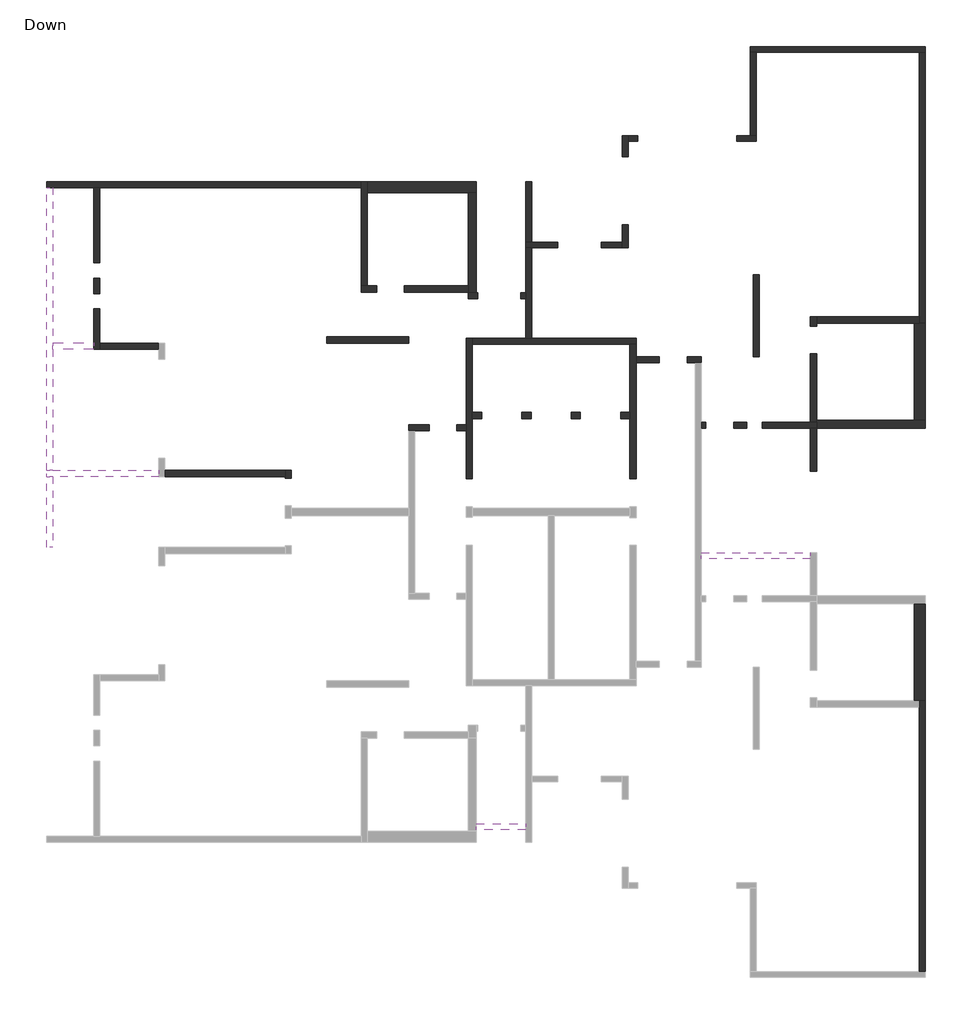
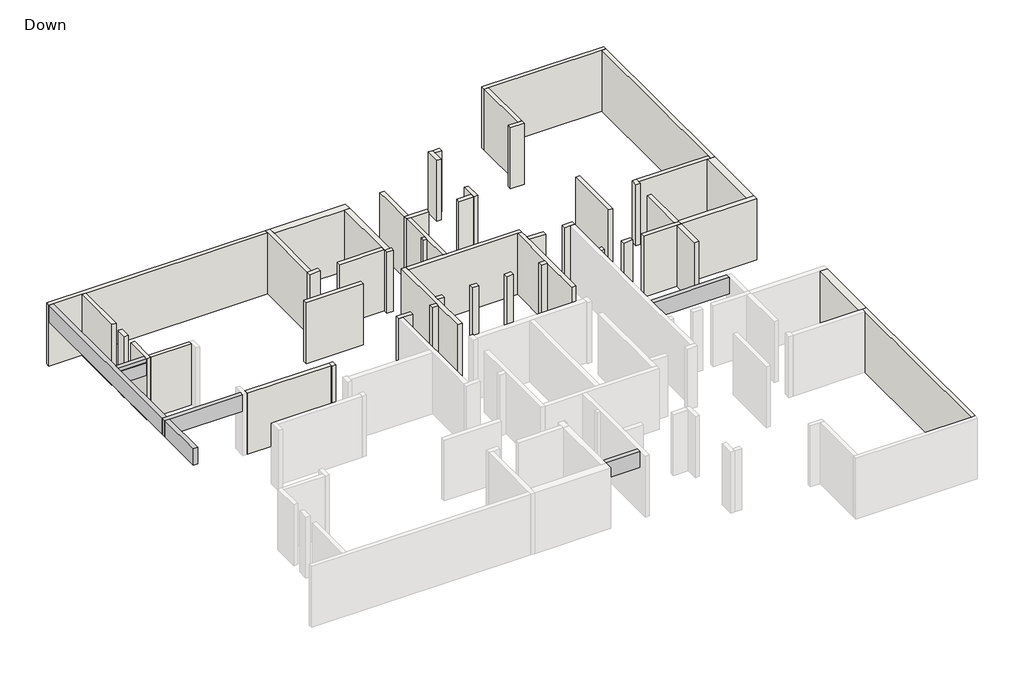
# One storey, part 2 of 2: 49 walls, 6 beams.
# Revit data of these elements (continued)
# Element 5 (IfcBeam, "Concrete Rectengular Beam : 20/80") (continued)
#   Comments = ""
#   Mark = "B8"
#   SOFiSTiK_AMG_Comments = ""
#   SOFiSTiK_AMG_Scheduled = yes
#   SOFiSTiK_AMG_Adjusted = yes
#   Structural Material = Concrete
#   Phase Created = New Construction
#   Materials on its faces: "Concrete"
# Element 6 (IfcBeam, "Concrete Rectengular Beam : 20/80")
#   Comments = ""
#   Mark = "B9"
#   SOFiSTiK_AMG_Comments = ""
#   SOFiSTiK_AMG_Scheduled = yes
#   SOFiSTiK_AMG_Adjusted = yes
#   Structural Material = Concrete
#   Phase Created = New Construction
#   Materials on its faces: "Concrete"
# Element 7 (IfcWall, "19")
#   Comments = ""
#   Mark = "W1"
#   SOFiSTiK_EdgeZones = "W1"
#   SOFiSTiK_AMG_Comments = ""
#   Top Offset = 0 cm
#   Base Offset = 0 cm
#   wall height = 300 cm
#   SOFiSTiK_AMG_Scheduled = yes
#   SOFiSTiK_AMG_Adjusted = yes
#   Phase Created = New Construction
#   Base Constraint = Down
#   Top Constraint = Typical Floor
#   Materials on its faces: "Concrete"
# Element 8 (IfcWall, "19")
#   Comments = ""
#   Mark = "W2"
#   SOFiSTiK_EdgeZones = "W2"
#   SOFiSTiK_AMG_Comments = ""
#   Top Offset = 0 cm
#   Base Offset = 0 cm
#   wall height = 300 cm
#   SOFiSTiK_AMG_Scheduled = yes
#   SOFiSTiK_AMG_Adjusted = yes
#   Phase Created = New Construction
#   Base Constraint = Down
#   Top Constraint = Typical Floor
#   Materials on its faces: "Concrete"
# Element 9 (IfcWall, "19")
#   Comments = ""
#   Mark = "W3"
#   SOFiSTiK_EdgeZones = "W3"
#   SOFiSTiK_AMG_Comments = ""
#   Top Offset = 0 cm
#   Base Offset = 0 cm
#   wall height = 300 cm
#   SOFiSTiK_AMG_Scheduled = yes
#   SOFiSTiK_AMG_Adjusted = yes
#   Phase Created = New Construction
#   Base Constraint = Down
#   Top Constraint = Typical Floor
#   Materials on its faces: "Concrete"
# Element 10 (IfcWall, "19")
#   Comments = ""
#   Mark = "W4"
#   SOFiSTiK_EdgeZones = "W4"
#   SOFiSTiK_AMG_Comments = ""
#   Top Offset = 0 cm
#   Base Offset = 0 cm
#   wall height = 300 cm
#   SOFiSTiK_AMG_Scheduled = yes
#   SOFiSTiK_AMG_Adjusted = yes
#   Phase Created = New Construction
#   Base Constraint = Down
#   Top Constraint = Typical Floor
#   Materials on its faces: "Concrete"
# Element 11 (IfcWall, "19")
#   Comments = ""
#   Mark = "W5"
#   SOFiSTiK_EdgeZones = "W5"
#   SOFiSTiK_AMG_Comments = ""
#   Top Offset = 0 cm
#   Base Offset = 0 cm
#   wall height = 300 cm
#   SOFiSTiK_AMG_Scheduled = yes
#   SOFiSTiK_AMG_Adjusted = yes
#   Phase Created = New Construction
#   Base Constraint = Down
#   Top Constraint = Typical Floor
#   Materials on its faces: "Concrete"
# Element 12 (IfcWall, "19")
#   Comments = ""
#   Mark = "W6"
#   SOFiSTiK_EdgeZones = "W6"
#   SOFiSTiK_AMG_Comments = ""
#   Top Offset = 0 cm
#   Base Offset = 0 cm
#   wall height = 300 cm
#   SOFiSTiK_AMG_Scheduled = yes
#   SOFiSTiK_AMG_Adjusted = yes
#   Phase Created = New Construction
#   Base Constraint = Down
#   Top Constraint = Typical Floor
#   Materials on its faces: "Concrete"
# Element 13 (IfcWall, "19")
#   Comments = ""
#   Mark = "W7"
#   SOFiSTiK_EdgeZones = "W7"
#   SOFiSTiK_AMG_Comments = ""
#   Top Offset = 0 cm
#   Base Offset = 0 cm
#   wall height = 300 cm
#   SOFiSTiK_AMG_Scheduled = yes
#   SOFiSTiK_AMG_Adjusted = yes
#   Phase Created = New Construction
#   Base Constraint = Down
#   Top Constraint = Typical Floor
#   Materials on its faces: "Concrete"
# Element 14 (IfcWall, "19")
#   Comments = ""
#   Mark = "W8"
#   SOFiSTiK_EdgeZones = "W8"
#   SOFiSTiK_AMG_Comments = ""
#   Top Offset = 0 cm
#   Base Offset = 0 cm
#   wall height = 300 cm
#   SOFiSTiK_AMG_Scheduled = yes
#   SOFiSTiK_AMG_Adjusted = yes
#   Phase Created = New Construction
#   Base Constraint = Down
#   Top Constraint = Typical Floor
#   Materials on its faces: "Concrete"
# Element 15 (IfcWall, "19")
#   Comments = ""
#   Mark = "W9"
#   SOFiSTiK_EdgeZones = "W9"
#   SOFiSTiK_AMG_Comments = ""
#   Top Offset = 0 cm
#   Base Offset = 0 cm
#   wall height = 300 cm
#   SOFiSTiK_AMG_Scheduled = yes
#   SOFiSTiK_AMG_Adjusted = yes
#   Phase Created = New Construction
#   Base Constraint = Down
#   Top Constraint = Typical Floor
#   Materials on its faces: "Concrete"
# Element 16 (IfcWall, "19")
#   Comments = ""
#   Mark = "W10"
#   SOFiSTiK_EdgeZones = "W10"
#   SOFiSTiK_AMG_Comments = ""
#   Top Offset = 0 cm
#   Base Offset = 0 cm
#   wall height = 300 cm
#   SOFiSTiK_AMG_Scheduled = yes
#   SOFiSTiK_AMG_Adjusted = yes
#   Phase Created = New Construction
#   Base Constraint = Down
#   Top Constraint = Typical Floor
#   Materials on its faces: "Concrete"
# Element 17 (IfcWall, "19")
#   Comments = ""
#   Mark = "W11"
#   SOFiSTiK_EdgeZones = "W11"
#   SOFiSTiK_AMG_Comments = ""
#   Top Offset = 0 cm
#   Base Offset = 0 cm
#   wall height = 300 cm
#   SOFiSTiK_AMG_Scheduled = yes
#   SOFiSTiK_AMG_Adjusted = yes
#   Phase Created = New Construction
#   Base Constraint = Down
#   Top Constraint = Typical Floor
#   Materials on its faces: "Concrete"
# Element 18 (IfcWall, "19")
#   Comments = ""
#   Mark = "W12"
#   SOFiSTiK_EdgeZones = "W12"
#   SOFiSTiK_AMG_Comments = ""
#   Top Offset = 0 cm
#   Base Offset = 0 cm
#   wall height = 300 cm
#   SOFiSTiK_AMG_Scheduled = yes
#   SOFiSTiK_AMG_Adjusted = yes
#   Phase Created = New Construction
#   Base Constraint = Down
#   Top Constraint = Typical Floor
#   Materials on its faces: "Concrete"
# Element 19 (IfcWall, "19")
#   Comments = ""
#   Mark = "W13"
#   SOFiSTiK_EdgeZones = "W13"
#   SOFiSTiK_AMG_Comments = ""
#   Top Offset = 0 cm
#   Base Offset = 0 cm
#   wall height = 300 cm
#   SOFiSTiK_AMG_Scheduled = yes
#   SOFiSTiK_AMG_Adjusted = yes
#   Phase Created = New Construction
#   Base Constraint = Down
#   Top Constraint = Typical Floor
#   Materials on its faces: "Concrete"
# Element 20 (IfcWall, "19")
#   Comments = ""
#   Mark = "W14"
#   SOFiSTiK_EdgeZones = "W14"
#   SOFiSTiK_AMG_Comments = ""
#   Top Offset = 0 cm
#   Base Offset = 0 cm
#   wall height = 300 cm
#   SOFiSTiK_AMG_Scheduled = yes
#   SOFiSTiK_AMG_Adjusted = yes
#   Phase Created = New Construction
#   Base Constraint = Down
#   Top Constraint = Typical Floor
#   Materials on its faces: "Concrete"
# Element 21 (IfcWall, "19")
#   Comments = ""
#   Mark = "W15"
#   SOFiSTiK_EdgeZones = "W15"
#   SOFiSTiK_AMG_Comments = ""
#   Top Offset = 0 cm
#   Base Offset = 0 cm
#   wall height = 300 cm
#   SOFiSTiK_AMG_Scheduled = yes
#   SOFiSTiK_AMG_Adjusted = yes
#   Phase Created = New Construction
#   Base Constraint = Down
#   Top Constraint = Typical Floor
#   Materials on its faces: "Concrete"
# Element 22 (IfcWall, "19")
#   Comments = ""
#   Mark = "W18"
#   SOFiSTiK_EdgeZones = "W18"
#   SOFiSTiK_AMG_Comments = ""
#   Top Offset = 0 cm
#   Base Offset = 0 cm
#   wall height = 300 cm
#   SOFiSTiK_AMG_Scheduled = yes
#   SOFiSTiK_AMG_Adjusted = yes
#   Phase Created = New Construction
#   Base Constraint = Down
#   Top Constraint = Typical Floor
#   Materials on its faces: "Concrete"
# Element 23 (IfcWall, "19")
#   Comments = ""
#   Mark = "W20"
#   SOFiSTiK_EdgeZones = "W20"
#   SOFiSTiK_AMG_Comments = ""
#   Top Offset = 0 cm
#   Base Offset = 0 cm
#   wall height = 300 cm
#   SOFiSTiK_AMG_Scheduled = yes
#   SOFiSTiK_AMG_Adjusted = yes
#   Phase Created = New Construction
#   Base Constraint = Down
#   Top Constraint = Typical Floor
#   Materials on its faces: "Concrete"
# Element 24 (IfcWall, "19")
#   Comments = ""
#   Mark = "W21"
#   SOFiSTiK_EdgeZones = "W21"
#   SOFiSTiK_AMG_Comments = ""
#   Top Offset = 0 cm
#   Base Offset = 0 cm
#   wall height = 300 cm
#   SOFiSTiK_AMG_Scheduled = yes
#   SOFiSTiK_AMG_Adjusted = yes
#   Phase Created = New Construction
#   Base Constraint = Down
#   Top Constraint = Typical Floor
#   Materials on its faces: "Concrete"
# Element 25 (IfcWall, "19")
#   Comments = ""
#   Mark = "W22"
#   SOFiSTiK_EdgeZones = "W22"
#   SOFiSTiK_AMG_Comments = ""
#   Top Offset = 0 cm
#   Base Offset = 0 cm
#   wall height = 300 cm
#   SOFiSTiK_AMG_Scheduled = yes
#   SOFiSTiK_AMG_Adjusted = yes
#   Phase Created = New Construction
#   Base Constraint = Down
#   Top Constraint = Typical Floor
#   Materials on its faces: "Concrete"
# Element 26 (IfcWall, "19")
#   Comments = ""
#   Mark = "W36"
#   SOFiSTiK_EdgeZones = "W36"
#   SOFiSTiK_AMG_Comments = ""
#   Top Offset = 0 cm
#   Base Offset = 0 cm
#   wall height = 300 cm
#   SOFiSTiK_AMG_Scheduled = yes
#   SOFiSTiK_AMG_Adjusted = yes
#   Phase Created = New Construction
#   Base Constraint = Down
#   Top Constraint = Typical Floor
#   Materials on its faces: "Concrete"
# Element 27 (IfcWall, "20")
#   Comments = ""
#   Mark = "W44"
#   SOFiSTiK_EdgeZones = "W44"
#   SOFiSTiK_AMG_Comments = ""
#   Top Offset = 0 cm
#   Base Offset = 0 cm
#   wall height = 300 cm
#   SOFiSTiK_AMG_Scheduled = yes
#   SOFiSTiK_AMG_Adjusted = yes
#   Phase Created = New Construction
#   Base Constraint = Down
#   Top Constraint = Typical Floor
#   Materials on its faces: "Concrete"
# Element 28 (IfcWall, "20")
#   Comments = ""
#   Mark = "W45"
#   SOFiSTiK_EdgeZones = "W45"
#   SOFiSTiK_AMG_Comments = ""
#   Top Offset = 0 cm
#   Base Offset = 0 cm
#   wall height = 300 cm
#   SOFiSTiK_AMG_Scheduled = yes
#   SOFiSTiK_AMG_Adjusted = yes
#   Phase Created = New Construction
#   Base Constraint = Down
#   Top Constraint = Typical Floor
#   Materials on its faces: "Concrete"
# Element 29 (IfcWall, "20")
#   Comments = ""
#   Mark = "W46"
#   SOFiSTiK_EdgeZones = "W46"
#   SOFiSTiK_AMG_Comments = ""
#   Top Offset = 0 cm
#   Base Offset = 0 cm
#   wall height = 300 cm
#   SOFiSTiK_AMG_Scheduled = yes
#   SOFiSTiK_AMG_Adjusted = yes
#   Phase Created = New Construction
#   Base Constraint = Down
#   Top Constraint = Typical Floor
#   Materials on its faces: "Concrete"
# Element 30 (IfcWall, "20")
#   Comments = ""
#   Mark = "W47"
#   SOFiSTiK_EdgeZones = "W47"
#   SOFiSTiK_AMG_Comments = ""
#   Top Offset = 0 cm
#   Base Offset = 0 cm
#   wall height = 300 cm
#   SOFiSTiK_AMG_Scheduled = yes
#   SOFiSTiK_AMG_Adjusted = yes
#   Phase Created = New Construction
#   Base Constraint = Down
#   Top Constraint = Typical Floor
#   Materials on its faces: "Concrete"
# Element 31 (IfcWall, "20")
#   Comments = ""
#   Mark = "W48"
#   SOFiSTiK_EdgeZones = "W48"
#   SOFiSTiK_AMG_Comments = ""
#   Top Offset = 0 cm
#   Base Offset = 0 cm
#   wall height = 300 cm
#   SOFiSTiK_AMG_Scheduled = yes
#   SOFiSTiK_AMG_Adjusted = yes
#   Phase Created = New Construction
#   Base Constraint = Down
#   Top Constraint = Typical Floor
#   Materials on its faces: "Concrete"
# Element 32 (IfcWall, "20")
#   Comments = ""
#   Mark = "W49"
#   SOFiSTiK_EdgeZones = "W49"
#   SOFiSTiK_AMG_Comments = ""
#   Top Offset = 0 cm
#   Base Offset = 0 cm
#   wall height = 300 cm
#   SOFiSTiK_AMG_Scheduled = yes
#   SOFiSTiK_AMG_Adjusted = yes
#   Phase Created = New Construction
#   Base Constraint = Down
#   Top Constraint = Typical Floor
#   Materials on its faces: "Concrete"
# Element 33 (IfcWall, "20")
#   Comments = ""
#   Mark = "W51"
#   SOFiSTiK_EdgeZones = "W51"
#   SOFiSTiK_AMG_Comments = ""
#   Top Offset = 0 cm
#   Base Offset = 0 cm
#   wall height = 300 cm
#   SOFiSTiK_AMG_Scheduled = yes
#   SOFiSTiK_AMG_Adjusted = yes
#   Phase Created = New Construction
#   Base Constraint = Down
#   Top Constraint = Typical Floor
#   Materials on its faces: "Concrete"
# Element 34 (IfcWall, "20")
#   Comments = ""
#   Mark = "W52"
#   SOFiSTiK_EdgeZones = "W52"
#   SOFiSTiK_AMG_Comments = ""
#   Top Offset = 0 cm
#   Base Offset = 0 cm
#   wall height = 300 cm
#   SOFiSTiK_AMG_Scheduled = yes
#   SOFiSTiK_AMG_Adjusted = yes
#   Phase Created = New Construction
#   Base Constraint = Down
#   Top Constraint = Typical Floor
#   Materials on its faces: "Concrete"
# Element 35 (IfcWall, "20")
#   Comments = ""
#   Mark = "W53"
#   SOFiSTiK_EdgeZones = "W53"
#   SOFiSTiK_AMG_Comments = ""
#   Top Offset = 0 cm
#   Base Offset = 0 cm
#   wall height = 300 cm
#   SOFiSTiK_AMG_Scheduled = yes
#   SOFiSTiK_AMG_Adjusted = yes
#   Phase Created = New Construction
#   Base Constraint = Down
#   Top Constraint = Typical Floor
#   Materials on its faces: "Concrete"
# Element 36 (IfcWall, "20")
#   Comments = ""
#   Mark = "W54"
#   SOFiSTiK_EdgeZones = "W54"
#   SOFiSTiK_AMG_Comments = ""
#   Top Offset = 0 cm
#   Base Offset = 0 cm
#   wall height = 300 cm
#   SOFiSTiK_AMG_Scheduled = yes
#   SOFiSTiK_AMG_Adjusted = yes
#   Phase Created = New Construction
#   Base Constraint = Down
#   Top Constraint = Typical Floor
#   Materials on its faces: "Concrete"
# Element 37 (IfcWall, "20")
#   Comments = ""
#   Mark = "W56"
#   SOFiSTiK_EdgeZones = "W56"
#   SOFiSTiK_AMG_Comments = ""
#   Top Offset = 0 cm
#   Base Offset = 0 cm
#   wall height = 300 cm
#   SOFiSTiK_AMG_Scheduled = yes
#   SOFiSTiK_AMG_Adjusted = yes
#   Phase Created = New Construction
#   Base Constraint = Down
#   Top Constraint = Typical Floor
#   Materials on its faces: "Concrete"
# Element 38 (IfcWall, "20")
#   Comments = ""
#   Mark = "W57"
#   SOFiSTiK_EdgeZones = "W57"
#   SOFiSTiK_AMG_Comments = ""
#   Top Offset = 0 cm
#   Base Offset = 0 cm
#   wall height = 300 cm
#   SOFiSTiK_AMG_Scheduled = yes
#   SOFiSTiK_AMG_Adjusted = yes
#   Phase Created = New Construction
#   Base Constraint = Down
#   Top Constraint = Typical Floor
#   Materials on its faces: "Concrete"
# Element 39 (IfcWall, "20")
#   Comments = ""
#   Mark = "W62"
#   SOFiSTiK_EdgeZones = "W62"
#   SOFiSTiK_AMG_Comments = ""
#   Top Offset = 0 cm
#   Base Offset = 0 cm
#   wall height = 300 cm
#   SOFiSTiK_AMG_Scheduled = yes
#   SOFiSTiK_AMG_Adjusted = yes
#   Phase Created = New Construction
#   Base Constraint = Down
#   Top Constraint = Typical Floor
#   Materials on its faces: "Concrete"
# Element 40 (IfcWall, "20")
#   Comments = ""
#   Mark = "W63"
#   SOFiSTiK_EdgeZones = "W63"
#   SOFiSTiK_AMG_Comments = ""
#   Top Offset = 0 cm
#   Base Offset = 0 cm
#   wall height = 300 cm
#   SOFiSTiK_AMG_Scheduled = yes
#   SOFiSTiK_AMG_Adjusted = yes
#   Phase Created = New Construction
#   Base Constraint = Down
#   Top Constraint = Typical Floor
#   Materials on its faces: "Concrete"
# Element 41 (IfcWall, "20")
#   Comments = ""
#   Mark = "W64"
#   SOFiSTiK_EdgeZones = "W64"
#   SOFiSTiK_AMG_Comments = ""
#   Top Offset = 0 cm
#   Base Offset = 0 cm
#   wall height = 300 cm
#   SOFiSTiK_AMG_Scheduled = yes
#   SOFiSTiK_AMG_Adjusted = yes
#   Phase Created = New Construction
#   Base Constraint = Down
#   Top Constraint = Typical Floor
#   Materials on its faces: "Concrete"
# Element 42 (IfcWall, "20")
#   Comments = ""
#   Mark = "W65"
#   SOFiSTiK_EdgeZones = "W65"
#   SOFiSTiK_AMG_Comments = ""
#   Top Offset = 0 cm
#   Base Offset = 0 cm
#   wall height = 300 cm
#   SOFiSTiK_AMG_Scheduled = yes
#   SOFiSTiK_AMG_Adjusted = yes
#   Phase Created = New Construction
#   Base Constraint = Down
#   Top Constraint = Typical Floor
#   Materials on its faces: "Concrete"
# Element 43 (IfcWall, "20")
#   Comments = ""
#   Mark = "W66"
#   SOFiSTiK_EdgeZones = "W66"
#   SOFiSTiK_AMG_Comments = ""
#   Top Offset = 0 cm
#   Base Offset = 0 cm
#   wall height = 300 cm
#   SOFiSTiK_AMG_Scheduled = yes
#   SOFiSTiK_AMG_Adjusted = yes
#   Phase Created = New Construction
#   Base Constraint = Down
#   Top Constraint = Typical Floor
#   Materials on its faces: "Concrete"
# Element 44 (IfcWall, "20")
#   Comments = ""
#   Mark = "W68"
#   SOFiSTiK_EdgeZones = "W68"
#   SOFiSTiK_AMG_Comments = "Too Short /"
#   Top Offset = 0 cm
#   Base Offset = 0 cm
#   wall height = 300 cm
#   SOFiSTiK_AMG_Scheduled = yes
#   SOFiSTiK_AMG_Adjusted = yes
#   Phase Created = New Construction
#   Base Constraint = Down
#   Top Constraint = Typical Floor
#   Materials on its faces: "Concrete"
# Element 45 (IfcWall, "20")
#   Comments = ""
#   Mark = "W69"
#   SOFiSTiK_EdgeZones = "W69"
#   SOFiSTiK_AMG_Comments = ""
#   Top Offset = 0 cm
#   Base Offset = 0 cm
#   wall height = 300 cm
#   SOFiSTiK_AMG_Scheduled = yes
#   SOFiSTiK_AMG_Adjusted = yes
#   Phase Created = New Construction
#   Base Constraint = Down
#   Top Constraint = Typical Floor
#   Materials on its faces: "Concrete"
# Element 46 (IfcWall, "20")
#   Comments = ""
#   Mark = "W70"
#   SOFiSTiK_EdgeZones = "W70"
#   SOFiSTiK_AMG_Comments = ""
#   Top Offset = 0 cm
#   Base Offset = 0 cm
#   wall height = 300 cm
#   SOFiSTiK_AMG_Scheduled = yes
#   SOFiSTiK_AMG_Adjusted = yes
#   Phase Created = New Construction
#   Base Constraint = Down
#   Top Constraint = Typical Floor
#   Materials on its faces: "Concrete"
# Element 47 (IfcWall, "20")
#   Comments = ""
#   Mark = "W71"
#   SOFiSTiK_EdgeZones = "W71"
#   SOFiSTiK_AMG_Comments = ""
#   Top Offset = 0 cm
#   Base Offset = 0 cm
#   wall height = 300 cm
#   SOFiSTiK_AMG_Scheduled = yes
#   SOFiSTiK_AMG_Adjusted = yes
#   Phase Created = New Construction
#   Base Constraint = Down
#   Top Constraint = Typical Floor
#   Materials on its faces: "Concrete"
# Element 48 (IfcWall, "20")
#   Comments = ""
#   Mark = "W72"
#   SOFiSTiK_EdgeZones = "W72"
#   SOFiSTiK_AMG_Comments = ""
#   Top Offset = 0 cm
#   Base Offset = 0 cm
#   wall height = 300 cm
#   SOFiSTiK_AMG_Scheduled = yes
#   SOFiSTiK_AMG_Adjusted = yes
#   Phase Created = New Construction
#   Base Constraint = Down
#   Top Constraint = Typical Floor
#   Materials on its faces: "Concrete"
# Element 49 (IfcWall, "20")
#   Comments = ""
#   Mark = "W73"
#   SOFiSTiK_EdgeZones = "W73"
#   SOFiSTiK_AMG_Comments = ""
#   Top Offset = 0 cm
#   Base Offset = 0 cm
#   wall height = 300 cm
#   SOFiSTiK_AMG_Scheduled = yes
#   SOFiSTiK_AMG_Adjusted = yes
#   Phase Created = New Construction
#   Base Constraint = Down
#   Top Constraint = Typical Floor
#   Materials on its faces: "Concrete"
# Element 50 (IfcWall, "20")
#   Comments = ""
#   Mark = "W74"
#   SOFiSTiK_EdgeZones = "W74"
#   SOFiSTiK_AMG_Comments = ""
#   Top Offset = 0 cm
#   Base Offset = 0 cm
#   wall height = 300 cm
#   SOFiSTiK_AMG_Scheduled = yes
#   SOFiSTiK_AMG_Adjusted = yes
#   Phase Created = New Construction
#   Base Constraint = Down
#   Top Constraint = Typical Floor
#   Materials on its faces: "Concrete"
# Element 51 (IfcWall, "25")
#   Comments = ""
#   Mark = "W101"
#   SOFiSTiK_EdgeZones = "W101"
#   SOFiSTiK_AMG_Comments = ""
#   Top Offset = 0 cm
#   Base Offset = 0 cm
#   wall height = 300 cm
#   SOFiSTiK_AMG_Scheduled = yes
#   SOFiSTiK_AMG_Adjusted = yes
#   Phase Created = New Construction
#   Base Constraint = Down
#   Top Constraint = Typical Floor
#   Materials on its faces: "Concrete"
# Element 52 (IfcWall, "25")
#   Comments = ""
#   Mark = "W104"
#   SOFiSTiK_EdgeZones = "W104"
#   SOFiSTiK_AMG_Comments = ""
#   Top Offset = 0 cm
#   Base Offset = 0 cm
#   wall height = 300 cm
#   SOFiSTiK_AMG_Scheduled = yes
#   SOFiSTiK_AMG_Adjusted = yes
#   Phase Created = New Construction
#   Base Constraint = Down
#   Top Constraint = Typical Floor
#   Materials on its faces: "Concrete"
# Element 53 (IfcWall, "35")
#   Comments = ""
#   Mark = "W108"
#   SOFiSTiK_EdgeZones = "W108"
#   SOFiSTiK_AMG_Comments = ""
#   Top Offset = 0 cm
#   Base Offset = 0 cm
#   wall height = 300 cm
#   SOFiSTiK_AMG_Scheduled = yes
#   SOFiSTiK_AMG_Adjusted = yes
#   Phase Created = New Construction
#   Base Constraint = Down
#   Top Constraint = Typical Floor
#   Materials on its faces: "Concrete"
# Element 54 (IfcWall, "35")
#   Comments = ""
#   Mark = "W109"
#   SOFiSTiK_EdgeZones = "W109"
#   SOFiSTiK_AMG_Comments = ""
#   Top Offset = 0 cm
#   Base Offset = 0 cm
#   wall height = 300 cm
#   SOFiSTiK_AMG_Scheduled = yes
#   SOFiSTiK_AMG_Adjusted = yes
#   Phase Created = New Construction
#   Base Constraint = Down
#   Top Constraint = Typical Floor
#   Materials on its faces: "Concrete"
# Element 55 (IfcWall, "35")
#   Comments = ""
#   Mark = "W111"
#   SOFiSTiK_EdgeZones = "W111"
#   SOFiSTiK_AMG_Comments = ""
#   Top Offset = 0 cm
#   Base Offset = 0 cm
#   wall height = 300 cm
#   SOFiSTiK_AMG_Scheduled = yes
#   SOFiSTiK_AMG_Adjusted = yes
#   Phase Created = New Construction
#   Base Constraint = Down
#   Top Constraint = Typical Floor
#   Materials on its faces: "Concrete"
# Materials
#   "Concrete": class "Concrete", colour RGB 192 192 192, transparency 0, Keynote = "01000", Description = "Cast-in-place concrete", Cost = 0
